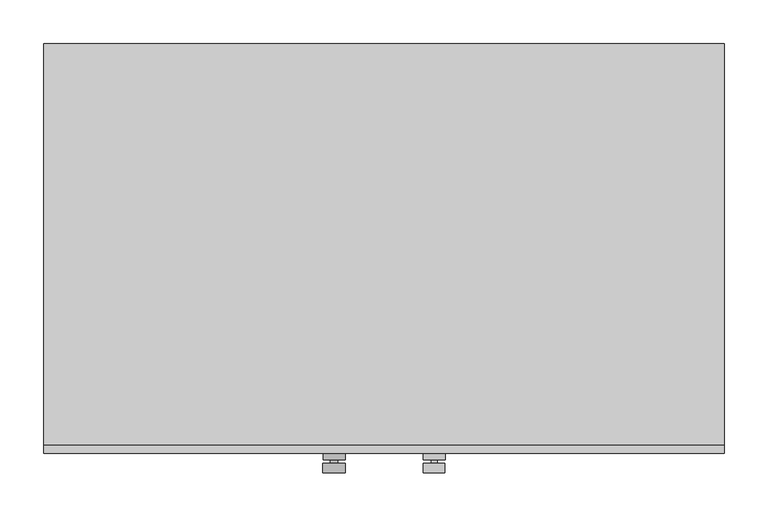
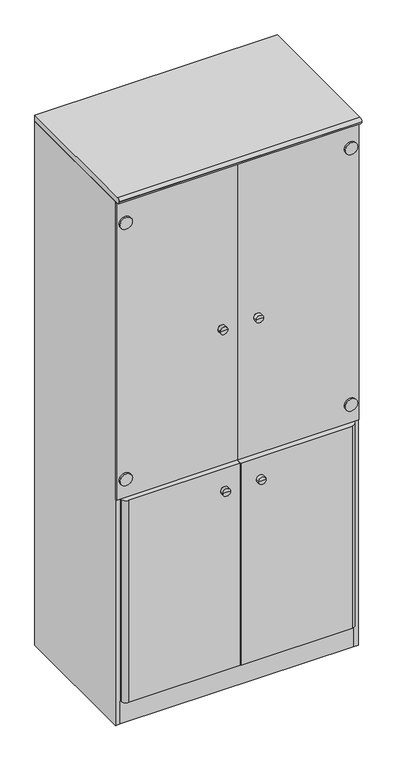
"""IFC4 building model written with IfcOpenShell, lengths in millimetres: furniture geometry, 书柜5 : W780*D450*H1800mm."""

from ifc_helpers import new_model, si_unit, point, frame, frame_2d, origin, origin_with_axes, place, context, project, spatial, polyline, circle_curve, trimmed, segment, composite_curve, outline, extrude, source, transform, mapped, element, save
from ifc_brep_helpers import plane_surface, cylinder_surface, advanced_brep


def furniture_aa1a75c8(model_context):
    return source(origin(), model_context, "Body", "SolidModel", [
        extrude(outline(composite_curve([segment(polyline([(-246.5557266, 1800.0), (214.2249346, 1800.0), (214.2249346, 1780.00298), (-246.553178, 1780.00298)]), True, "CONTINUOUS"), segment(trimmed(circle_curve(frame_2d((-246.553178, 1789.2248674)), 9.2218874), [point((-246.553178, 1780.00298))], [point((-255.7750654, 1789.2248674))], False, "CARTESIAN"), True, "CONTINUOUS"), segment(polyline([(-255.7750654, 1789.2248674), (-255.7750654, 1790.7806612)]), True, "CONTINUOUS"), segment(trimmed(circle_curve(frame_2d((-246.5557266, 1790.7806612)), 9.2193388), [point((-255.7750654, 1790.7806612))], [point((-246.5557266, 1800.0))], False, "CARTESIAN"), True, "CONTINUOUS")], self_intersect=False)), frame((-390.267589, 0.0, 0.0), z_axis=(1.0, 0.0, 0.0), x_axis=(0.0, 1.0, 0.0)), (0.0, 0.0, 1.0), 780.0),
        extrude(outline(composite_curve([segment(trimmed(circle_curve(frame_2d((832.0298722, 361.9800403)), 20.0), [point((832.0298722, 381.9800403))], [point((832.0298722, 341.9800403))], False, "CARTESIAN"), True, "CONTINUOUS"), segment(trimmed(circle_curve(frame_2d((832.0298722, 361.9800403)), 20.0), [point((832.0298722, 341.9800403))], [point((832.0298722, 381.9800403))], False, "CARTESIAN"), True, "CONTINUOUS")], self_intersect=False)), frame((0.0, -246.5557266, 0.0), z_axis=(0.0, 1.0, 0.0), x_axis=(0.0, 0.0, 1.0)), (0.0, 0.0, 1.0), 5.7806612),
        extrude(outline(composite_curve([segment(trimmed(circle_curve(frame_2d((1702.9701278, 361.9800403)), 20.0), [point((1702.9701278, 381.9800403))], [point((1702.9701278, 341.9800403))], False, "CARTESIAN"), True, "CONTINUOUS"), segment(trimmed(circle_curve(frame_2d((1702.9701278, 361.9800403)), 20.0), [point((1702.9701278, 341.9800403))], [point((1702.9701278, 381.9800403))], False, "CARTESIAN"), True, "CONTINUOUS")], self_intersect=False)), frame((0.0, -246.5557266, 0.0), z_axis=(0.0, 1.0, 0.0), x_axis=(0.0, 0.0, 1.0)), (0.0, 0.0, 1.0), 5.7806612),
        extrude(outline(composite_curve([segment(trimmed(circle_curve(frame_2d((1702.9701278, -362.5152184)), 20.0), [point((1702.9701278, -382.5152184))], [point((1702.9701278, -342.5152184))], False, "CARTESIAN"), True, "CONTINUOUS"), segment(trimmed(circle_curve(frame_2d((1702.9701278, -362.5152184)), 20.0), [point((1702.9701278, -342.5152184))], [point((1702.9701278, -382.5152184))], False, "CARTESIAN"), True, "CONTINUOUS")], self_intersect=False)), frame((0.0, -246.5557266, 0.0), z_axis=(0.0, 1.0, 0.0), x_axis=(0.0, 0.0, 1.0)), (0.0, 0.0, 1.0), 5.7806612),
        extrude(outline(composite_curve([segment(trimmed(circle_curve(frame_2d((832.0298722, -362.5152184)), 20.0), [point((832.0298722, -382.5152184))], [point((832.0298722, -342.5152184))], False, "CARTESIAN"), True, "CONTINUOUS"), segment(trimmed(circle_curve(frame_2d((832.0298722, -362.5152184)), 20.0), [point((832.0298722, -342.5152184))], [point((832.0298722, -382.5152184))], False, "CARTESIAN"), True, "CONTINUOUS")], self_intersect=False)), frame((0.0, -246.5557266, 0.0), z_axis=(0.0, 1.0, 0.0), x_axis=(0.0, 0.0, 1.0)), (0.0, 0.0, 1.0), 5.7806612),
        extrude(outline(composite_curve([segment(polyline([(-375.3567854, -235.7750654), (-1.4459817, -235.7750654), (-1.4459817, -255.7750654), (-359.5899795, -255.7750654)]), True, "CONTINUOUS"), segment(trimmed(circle_curve(frame_2d((-359.5899795, -240.0082595)), 15.7668059), [point((-359.5899795, -255.7750654))], [point((-375.3567854, -240.0082595))], False, "CARTESIAN"), True, "CONTINUOUS"), segment(polyline([(-375.3567854, -240.0082595), (-375.3567854, -235.7750654)]), True, "CONTINUOUS")], self_intersect=False)), frame((0.0, 0.0, 80.0), z_axis=(0.0, 0.0, 1.0), x_axis=(1.0, 0.0, 0.0)), (0.0, 0.0, 1.0), 686.4),
        advanced_brep(
        [(-57.4433336, -240.7750654, 1241.1237815), (-53.4331008, -240.7750654, 1241.1237815), (-61.4535664, -240.7750654, 1241.1237815), (-69.9433336, -263.0203049, 1241.1237815), (-44.9433336, -263.0203049, 1241.1237815), (-57.4433336, -263.0203049, 1241.1237815), (-69.9433336, -251.699089, 1241.1237815), (-44.9433336, -251.699089, 1241.1237815), (-61.4535664, -251.699089, 1241.1237815), (-53.4331008, -251.699089, 1241.1237815)],
        [
            (0, 1),
            (1, 2, circle_curve(frame((-57.4433336, -240.7750654, 1241.1237815), z_axis=(0.0, 1.0, 0.0), x_axis=(1.0, 0.0, 0.0)), 4.0102328)),
            (2, 0),
            (2, 1, circle_curve(frame((-57.4433336, -240.7750654, 1241.1237815), z_axis=(0.0, 1.0, 0.0), x_axis=(1.0, 0.0, 0.0)), 4.0102328)),
            (3, 4, circle_curve(frame((-57.4433336, -263.0203049, 1241.1237815), z_axis=(0.0, -1.0, 0.0), x_axis=(1.0, 0.0, 0.0)), 12.5)),
            (4, 5),
            (5, 3),
            (4, 3, circle_curve(frame((-57.4433336, -263.0203049, 1241.1237815), z_axis=(0.0, -1.0, 0.0), x_axis=(1.0, 0.0, 0.0)), 12.5)),
            (6, 7, circle_curve(frame((-57.4433336, -251.699089, 1241.1237815), z_axis=(0.0, -1.0, 0.0), x_axis=(1.0, 0.0, 0.0)), 12.5)),
            (7, 4),
            (3, 6),
            (7, 6, circle_curve(frame((-57.4433336, -251.699089, 1241.1237815), z_axis=(0.0, -1.0, 0.0), x_axis=(1.0, 0.0, 0.0)), 12.5)),
            (8, 9, circle_curve(frame((-57.4433336, -251.699089, 1241.1237815), z_axis=(0.0, -1.0, 0.0), x_axis=(1.0, 0.0, 0.0)), 4.0102328)),
            (9, 7),
            (6, 8),
            (9, 8, circle_curve(frame((-57.4433336, -251.699089, 1241.1237815), z_axis=(0.0, -1.0, 0.0), x_axis=(1.0, 0.0, 0.0)), 4.0102328)),
            (1, 9),
            (8, 2),
        ],
        [
            plane_surface(frame((-57.4433336, -240.7750654, 1241.1237815), z_axis=(0.0, 1.0, 0.0), x_axis=(1.0, 0.0, 0.0))),
            plane_surface(frame((-57.4433336, -263.0203049, 1241.1237815), z_axis=(0.0, -1.0, 0.0), x_axis=(1.0, 0.0, 0.0))),
            cylinder_surface(frame((-57.4433336, -165.4689088, 1241.1237815), z_axis=(0.0, 1.0, 0.0), x_axis=(1.0, 0.0, 0.0)), 12.5),
            plane_surface(frame((-57.4433336, -251.699089, 1241.1237815), z_axis=(0.0, 1.0, 0.0), x_axis=(1.0, 0.0, 0.0))),
            cylinder_surface(frame((-57.4433336, -165.4689088, 1241.1237815), z_axis=(0.0, 1.0, 0.0), x_axis=(1.0, 0.0, 0.0)), 4.0102328),
        ],
        [
            (0, [[1, 2, 3]]),
            (0, [[-3, 4, -1]]),
            (1, [[5, 6, 7]]),
            (1, [[8, -7, -6]]),
            (2, [[9, 10, -5, 11]]),
            (2, [[12, -11, -8, -10]]),
            (3, [[13, 14, -9, 15]]),
            (3, [[16, -15, -12, -14]]),
            (4, [[-2, 17, -13, 18]]),
            (4, [[-4, -18, -16, -17]]),
        ],
    ),
        advanced_brep(
        [(60.8777058, -251.699089, 1241.1237815), (53.652176, -251.699089, 1241.1237815), (53.652176, -240.7750654, 1241.1237815), (60.8777058, -240.7750654, 1241.1237815), (69.7649409, -251.699089, 1241.1237815), (44.7649409, -251.699089, 1241.1237815), (69.7649409, -263.0203049, 1241.1237815), (44.7649409, -263.0203049, 1241.1237815), (57.2649409, -263.0203049, 1241.1237815), (57.2649409, -240.7750654, 1241.1237815)],
        [
            (0, 1, circle_curve(frame((57.2649409, -251.699089, 1241.1237815), z_axis=(0.0, 1.0, 0.0), x_axis=(-1.0, 0.0, 0.0)), 3.6127649)),
            (1, 2),
            (2, 3, circle_curve(frame((57.2649409, -240.7750654, 1241.1237815), z_axis=(0.0, -1.0, 0.0), x_axis=(-1.0, 0.0, 0.0)), 3.6127649)),
            (3, 0),
            (1, 0, circle_curve(frame((57.2649409, -251.699089, 1241.1237815), z_axis=(0.0, 1.0, 0.0), x_axis=(-1.0, 0.0, 0.0)), 3.6127649)),
            (3, 2, circle_curve(frame((57.2649409, -240.7750654, 1241.1237815), z_axis=(0.0, -1.0, 0.0), x_axis=(-1.0, 0.0, 0.0)), 3.6127649)),
            (4, 5, circle_curve(frame((57.2649409, -251.699089, 1241.1237815), z_axis=(0.0, 1.0, 0.0), x_axis=(-1.0, 0.0, 0.0)), 12.5)),
            (5, 1),
            (0, 4),
            (5, 4, circle_curve(frame((57.2649409, -251.699089, 1241.1237815), z_axis=(0.0, 1.0, 0.0), x_axis=(-1.0, 0.0, 0.0)), 12.5)),
            (6, 7, circle_curve(frame((57.2649409, -263.0203049, 1241.1237815), z_axis=(0.0, 1.0, 0.0), x_axis=(-1.0, 0.0, 0.0)), 12.5)),
            (7, 5),
            (4, 6),
            (7, 6, circle_curve(frame((57.2649409, -263.0203049, 1241.1237815), z_axis=(0.0, 1.0, 0.0), x_axis=(-1.0, 0.0, 0.0)), 12.5)),
            (8, 7),
            (6, 8),
            (2, 9),
            (9, 3),
        ],
        [
            cylinder_surface(frame((57.2649409, -165.4689088, 1241.1237815), z_axis=(0.0, -1.0, 0.0), x_axis=(-1.0, 0.0, 0.0)), 3.6127649),
            plane_surface(frame((57.2649409, -251.699089, 1241.1237815), z_axis=(0.0, 1.0, 0.0), x_axis=(-1.0, 0.0, 0.0))),
            cylinder_surface(frame((57.2649409, -165.4689088, 1241.1237815), z_axis=(0.0, -1.0, 0.0), x_axis=(-1.0, 0.0, 0.0)), 12.5),
            plane_surface(frame((57.2649409, -263.0203049, 1241.1237815), z_axis=(0.0, -1.0, 0.0), x_axis=(-1.0, 0.0, 0.0))),
            plane_surface(frame((57.2649409, -240.7750654, 1241.1237815), z_axis=(0.0, 1.0, 0.0), x_axis=(-1.0, 0.0, 0.0))),
        ],
        [
            (0, [[1, 2, 3, 4]]),
            (0, [[5, -4, 6, -2]]),
            (1, [[7, 8, -1, 9]]),
            (1, [[10, -9, -5, -8]]),
            (2, [[11, 12, -7, 13]]),
            (2, [[14, -13, -10, -12]]),
            (3, [[15, -11, 16]]),
            (3, [[-16, -14, -15]]),
            (4, [[-3, 17, 18]]),
            (4, [[-6, -18, -17]]),
        ],
    ),
        extrude(outline(polyline([(0.9108037, -235.7750654), (389.732411, -235.7750654), (389.732411, -240.7750654), (0.9108037, -240.7750654), (0.9108037, -235.7750654)])), frame((0.0, 0.0, 769.0), z_axis=(0.0, 0.0, 1.0), x_axis=(1.0, 0.0, 0.0)), (0.0, 0.0, 1.0), 1009.0),
        extrude(outline(polyline([(-1.0891963, -235.7750654), (-1.0891963, -240.7750654), (-390.267589, -240.7750654), (-390.267589, -235.7750654), (-1.0891963, -235.7750654)])), frame((0.0, 0.0, 769.0), z_axis=(0.0, 0.0, 1.0), x_axis=(1.0, 0.0, 0.0)), (0.0, 0.0, 1.0), 1009.0),
        extrude(outline(composite_curve([segment(polyline([(374.8216073, -235.7750654), (374.8216073, -240.0082595)]), True, "CONTINUOUS"), segment(trimmed(circle_curve(frame_2d((359.0548014, -240.0082595)), 15.7668059), [point((374.8216073, -240.0082595))], [point((359.0548014, -255.7750654))], False, "CARTESIAN"), True, "CONTINUOUS"), segment(polyline([(359.0548014, -255.7750654), (0.9108037, -255.7750654), (0.9108037, -235.7750654), (374.8216073, -235.7750654)]), True, "CONTINUOUS")], self_intersect=False)), frame((0.0, 0.0, 80.0), z_axis=(0.0, 0.0, 1.0), x_axis=(1.0, 0.0, 0.0)), (0.0, 0.0, 1.0), 686.4),
        extrude(outline(polyline([(374.8216073, -215.6693649), (-375.1783927, -215.6693649), (-375.1783927, 198.2249346), (374.8216073, 198.2249346), (374.8216073, -215.6693649)])), frame((0.0, 0.0, 749.2), z_axis=(0.0, 0.0, 1.0), x_axis=(1.0, 0.0, 0.0)), (0.0, 0.0, 1.0), 17.2),
        extrude(outline(polyline([(374.8216073, 198.2249346), (-375.1783927, 198.2249346), (-375.1783927, 204.2249346), (374.8216073, 204.2249346), (374.8216073, 198.2249346)])), origin_with_axes(), (0.0, 0.0, 1.0), 60.0),
        extrude(outline(polyline([(374.8216073, -215.6693649), (374.8216073, -235.7750654), (-375.1783927, -235.7750654), (-375.1783927, -215.6693649), (374.8216073, -215.6693649)])), origin_with_axes(), (0.0, 0.0, 1.0), 78.0),
        extrude(outline(polyline([(374.8216073, -215.6693649), (-375.1783927, -215.6693649), (-375.1783927, 214.2249346), (374.8216073, 214.2249346), (374.8216073, -215.6693649)])), frame((0.0, 0.0, 60.0), z_axis=(0.0, 0.0, 1.0), x_axis=(1.0, 0.0, 0.0)), (0.0, 0.0, 1.0), 18.0),
        extrude(outline(polyline([(374.8216073, 198.2249346), (-375.1783927, 198.2249346), (-375.1783927, 204.2249346), (374.8216073, 204.2249346), (374.8216073, 198.2249346)])), frame((0.0, 0.0, 78.0), z_axis=(0.0, 0.0, 1.0), x_axis=(1.0, 0.0, 0.0)), (0.0, 0.0, 1.0), 1702.0),
        advanced_brep(
        [(-57.6217263, -255.7750654, 701.1237815), (-53.4331008, -255.7750654, 701.1237815), (-61.8103517, -255.7750654, 701.1237815), (-70.300119, -278.0203049, 701.1237815), (-44.9433336, -278.0203049, 701.1237815), (-57.6217263, -278.0203049, 701.1237815), (-70.300119, -266.699089, 701.1237815), (-44.9433336, -266.699089, 701.1237815), (-61.8103517, -266.699089, 701.1237815), (-53.4331008, -266.699089, 701.1237815)],
        [
            (0, 1),
            (1, 2, circle_curve(frame((-57.6217263, -255.7750654, 701.1237815), z_axis=(0.0, 1.0, 0.0), x_axis=(1.0, 0.0, 0.0)), 4.1886255)),
            (2, 0),
            (2, 1, circle_curve(frame((-57.6217263, -255.7750654, 701.1237815), z_axis=(0.0, 1.0, 0.0), x_axis=(1.0, 0.0, 0.0)), 4.1886255)),
            (3, 4, circle_curve(frame((-57.6217263, -278.0203049, 701.1237815), z_axis=(0.0, -1.0, 0.0), x_axis=(1.0, 0.0, 0.0)), 12.6783927)),
            (4, 5),
            (5, 3),
            (4, 3, circle_curve(frame((-57.6217263, -278.0203049, 701.1237815), z_axis=(0.0, -1.0, 0.0), x_axis=(1.0, 0.0, 0.0)), 12.6783927)),
            (6, 7, circle_curve(frame((-57.6217263, -266.699089, 701.1237815), z_axis=(0.0, -1.0, 0.0), x_axis=(1.0, 0.0, 0.0)), 12.6783927)),
            (7, 4),
            (3, 6),
            (7, 6, circle_curve(frame((-57.6217263, -266.699089, 701.1237815), z_axis=(0.0, -1.0, 0.0), x_axis=(1.0, 0.0, 0.0)), 12.6783927)),
            (8, 9, circle_curve(frame((-57.6217263, -266.699089, 701.1237815), z_axis=(0.0, -1.0, 0.0), x_axis=(1.0, 0.0, 0.0)), 4.1886255)),
            (9, 7),
            (6, 8),
            (9, 8, circle_curve(frame((-57.6217263, -266.699089, 701.1237815), z_axis=(0.0, -1.0, 0.0), x_axis=(1.0, 0.0, 0.0)), 4.1886255)),
            (1, 9),
            (8, 2),
        ],
        [
            plane_surface(frame((-57.6217263, -255.7750654, 701.1237815), z_axis=(0.0, 1.0, 0.0), x_axis=(1.0, 0.0, 0.0))),
            plane_surface(frame((-57.6217263, -278.0203049, 701.1237815), z_axis=(0.0, -1.0, 0.0), x_axis=(1.0, 0.0, 0.0))),
            cylinder_surface(frame((-57.6217263, -180.4689088, 701.1237815), z_axis=(0.0, 1.0, 0.0), x_axis=(1.0, 0.0, 0.0)), 12.6783927),
            plane_surface(frame((-57.6217263, -266.699089, 701.1237815), z_axis=(0.0, 1.0, 0.0), x_axis=(1.0, 0.0, 0.0))),
            cylinder_surface(frame((-57.6217263, -180.4689088, 701.1237815), z_axis=(0.0, 1.0, 0.0), x_axis=(1.0, 0.0, 0.0)), 4.1886255),
        ],
        [
            (0, [[1, 2, 3]]),
            (0, [[-3, 4, -1]]),
            (1, [[5, 6, 7]]),
            (1, [[8, -7, -6]]),
            (2, [[9, 10, -5, 11]]),
            (2, [[12, -11, -8, -10]]),
            (3, [[13, 14, -9, 15]]),
            (3, [[16, -15, -12, -14]]),
            (4, [[-2, 17, -13, 18]]),
            (4, [[-4, -18, -16, -17]]),
        ],
    ),
        advanced_brep(
        [(60.5209204, -266.699089, 701.1237815), (53.652176, -266.699089, 701.1237815), (53.652176, -255.8777654, 701.1237815), (60.5209204, -255.8777654, 701.1237815), (69.4081555, -266.699089, 701.1237815), (44.7649409, -266.699089, 701.1237815), (69.4081555, -278.0203049, 701.1237815), (44.7649409, -278.0203049, 701.1237815), (57.0865482, -278.0203049, 701.1237815), (57.0865482, -255.8777654, 701.1237815)],
        [
            (0, 1, circle_curve(frame((57.0865482, -266.699089, 701.1237815), z_axis=(0.0, 1.0, 0.0), x_axis=(-1.0, 0.0, 0.0)), 3.4343722)),
            (1, 2),
            (2, 3, circle_curve(frame((57.0865482, -255.8777654, 701.1237815), z_axis=(0.0, -1.0, 0.0), x_axis=(-1.0, 0.0, 0.0)), 3.4343722)),
            (3, 0),
            (1, 0, circle_curve(frame((57.0865482, -266.699089, 701.1237815), z_axis=(0.0, 1.0, 0.0), x_axis=(-1.0, 0.0, 0.0)), 3.4343722)),
            (3, 2, circle_curve(frame((57.0865482, -255.8777654, 701.1237815), z_axis=(0.0, -1.0, 0.0), x_axis=(-1.0, 0.0, 0.0)), 3.4343722)),
            (4, 5, circle_curve(frame((57.0865482, -266.699089, 701.1237815), z_axis=(0.0, 1.0, 0.0), x_axis=(-1.0, 0.0, 0.0)), 12.3216073)),
            (5, 1),
            (0, 4),
            (5, 4, circle_curve(frame((57.0865482, -266.699089, 701.1237815), z_axis=(0.0, 1.0, 0.0), x_axis=(-1.0, 0.0, 0.0)), 12.3216073)),
            (6, 7, circle_curve(frame((57.0865482, -278.0203049, 701.1237815), z_axis=(0.0, 1.0, 0.0), x_axis=(-1.0, 0.0, 0.0)), 12.3216073)),
            (7, 5),
            (4, 6),
            (7, 6, circle_curve(frame((57.0865482, -278.0203049, 701.1237815), z_axis=(0.0, 1.0, 0.0), x_axis=(-1.0, 0.0, 0.0)), 12.3216073)),
            (8, 7),
            (6, 8),
            (2, 9),
            (9, 3),
        ],
        [
            cylinder_surface(frame((57.0865482, -180.4689088, 701.1237815), z_axis=(0.0, -1.0, 0.0), x_axis=(-1.0, 0.0, 0.0)), 3.4343722),
            plane_surface(frame((57.0865482, -266.699089, 701.1237815), z_axis=(0.0, 1.0, 0.0), x_axis=(-1.0, 0.0, 0.0))),
            cylinder_surface(frame((57.0865482, -180.4689088, 701.1237815), z_axis=(0.0, -1.0, 0.0), x_axis=(-1.0, 0.0, 0.0)), 12.3216073),
            plane_surface(frame((57.0865482, -278.0203049, 701.1237815), z_axis=(0.0, -1.0, 0.0), x_axis=(-1.0, 0.0, 0.0))),
            plane_surface(frame((57.0865482, -255.8777654, 701.1237815), z_axis=(0.0, 1.0, 0.0), x_axis=(-1.0, 0.0, 0.0))),
        ],
        [
            (0, [[1, 2, 3, 4]]),
            (0, [[5, -4, 6, -2]]),
            (1, [[7, 8, -1, 9]]),
            (1, [[10, -9, -5, -8]]),
            (2, [[11, 12, -7, 13]]),
            (2, [[14, -13, -10, -12]]),
            (3, [[15, -11, 16]]),
            (3, [[-16, -14, -15]]),
            (4, [[-3, 17, 18]]),
            (4, [[-6, -18, -17]]),
        ],
    ),
        extrude(outline(polyline([(374.8216073, 198.2249346), (374.8216073, -215.6693649), (-375.1783927, -215.6693649), (-375.1783927, 198.2249346), (374.8216073, 198.2249346)])), frame((0.0, 0.0, 1095.2666667), z_axis=(0.0, 0.0, 1.0), x_axis=(1.0, 0.0, 0.0)), (0.0, 0.0, 1.0), 18.0),
        extrude(outline(polyline([(374.8216073, 198.2249346), (374.8216073, -215.6693649), (-375.1783927, -215.6693649), (-375.1783927, 198.2249346), (374.8216073, 198.2249346)])), frame((0.0, 0.0, 1433.1333333), z_axis=(0.0, 0.0, 1.0), x_axis=(1.0, 0.0, 0.0)), (0.0, 0.0, 1.0), 18.0),
        extrude(outline(polyline([(-390.267589, 214.2249346), (-375.1783927, 214.2249346), (-375.1783927, -235.7750654), (-390.267589, -235.7750654), (-390.267589, 214.2249346)])), origin_with_axes(), (0.0, 0.0, 1.0), 1780.0),
        extrude(outline(polyline([(389.732411, 214.2249346), (389.732411, -235.7750654), (374.8216073, -235.7750654), (374.8216073, 214.2249346), (389.732411, 214.2249346)])), origin_with_axes(), (0.0, 0.0, 1.0), 1780.0),
    ])


if __name__ == "__main__":
    model = new_model("IFC4")
    model_context = context("Model", 3, world=origin())
    ifc_project = project(units=[si_unit("LENGTHUNIT", "METRE", prefix="MILLI")], contexts=[model_context])
    site = spatial("IfcSite", under=ifc_project)
    building = spatial("IfcBuilding", under=site)
    placement = place(None, origin())
    furniture_shape = furniture_aa1a75c8(model_context)
    element("IfcFurniture", 1, ObjectType="书柜5 : W780*D450*H1800mm", at=placement, inside=building, context=model_context, shape_type="MappedRepresentation", body=[
        mapped(furniture_shape, transform((0.0, 0.0, 0.0), x_axis=(1.0, 0.0, 0.0), y_axis=(0.0, 1.0, 0.0), z_axis=(0.0, 0.0, 1.0))),
    ])
    save(model, "model.ifc")

# Revit data of these elements
# Type "书柜5 : W780*D450*H1800mm"
#   W = 780 mm
#   H = 1800 mm
#   D = 450 mm
#   门板材质 = 木质面层(1)
#   搁板材质 = 白油漆
#   配件材质 = 金属 - 不锈钢，抛光
#   玻璃材质 = 玻璃
#   Manufacturer = ""
#   Model = ""
# Element 1 (IfcFurniture, "书柜5 : W780*D450*H1800mm")
#   Materials on its faces: "木质面层(1)", "金属 - 不锈钢，抛光", "白油漆", "玻璃"
# Materials
#   "木质面层(1)": class "木质", colour RGB 173 104 78, transparency 0
#   "白油漆": class "油漆", colour RGB 252 252 252, transparency 0
#   "金属 - 不锈钢，抛光": class "金属", colour RGB 236 239 239, transparency 0, Cost = 0
#   "玻璃": class "玻璃", colour RGB 0 128 192, transparency 0.9, Description = "钠钙玻璃", Cost = 0
